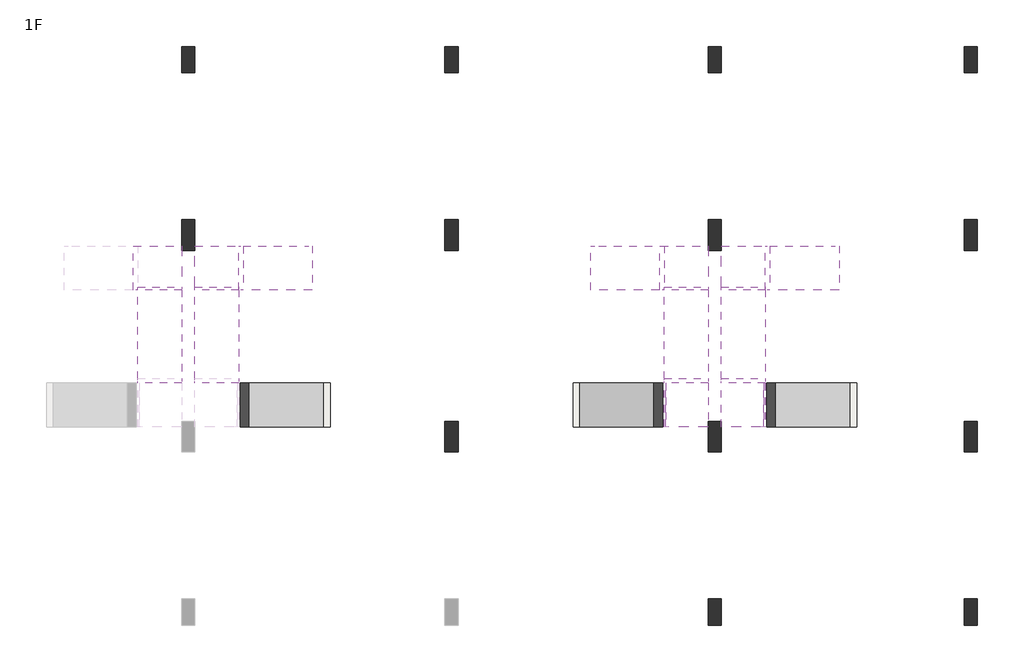
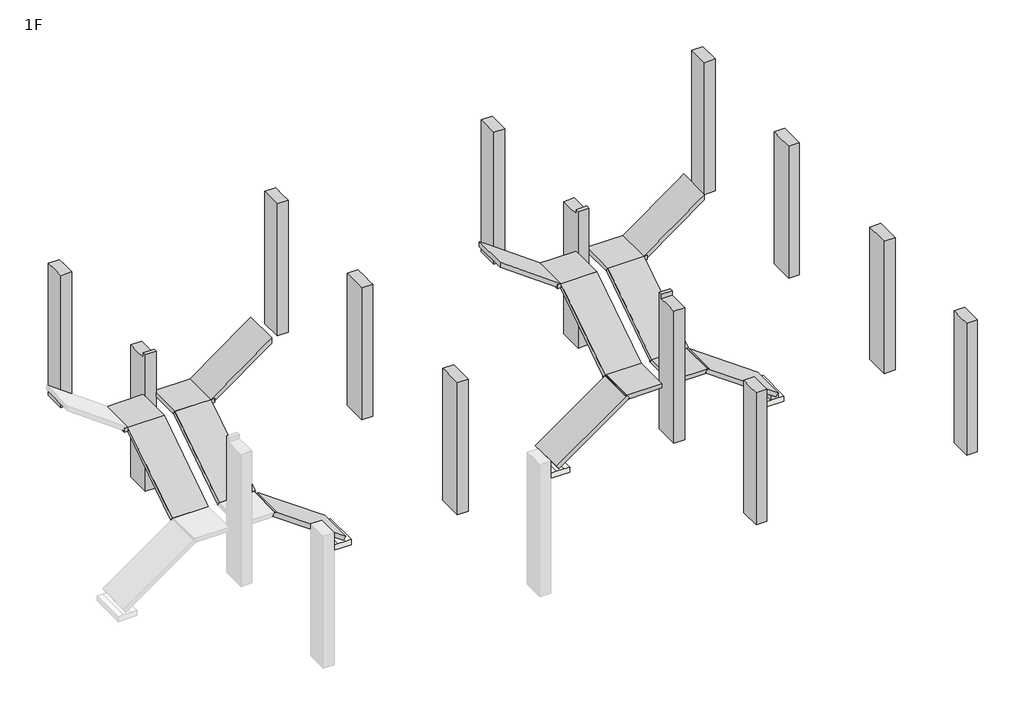
# One storey, part 2 of 2: 17 beams, 13 columns, 3 slabs.
"""IFC4 building model written with IfcOpenShell, lengths in millimetres."""

from ifc_helpers import new_model, si_unit, frame, origin, place, context, project, spatial, polyline, outline, extrude, faceted_brep, element, save

model = new_model("IFC4")

# Units and contexts
model_context = context("Model", 3, world=origin())
ifc_project = project(units=[si_unit("LENGTHUNIT", "METRE", prefix="MILLI")], contexts=[model_context])

# Site, building, storey
site = spatial("IfcSite", under=ifc_project)
building = spatial("IfcBuilding", under=site)
storey = spatial("IfcBuildingStorey", under=building, Name="1F", Elevation=30.0)

# Beams
placement = place(None, origin())
element("IfcBeam", 1, ObjectType="M_Concrete-Rectangular Beam : 1000x120", at=placement, inside=storey, context=model_context, shape_type="Brep", body=[
    faceted_brep([(16700.0000058, 7550.0000002, 2813.0), (17700.0000058, 7550.0000002, 2813.0), (17700.0000058, 7615.755173, 2712.6194379), (16700.0000058, 7615.755173, 2712.6194379), (16700.0000058, 5424.9999998, 1421.0), (16700.0000058, 5490.7551727, 1320.6194379), (17700.0000058, 5490.7551727, 1320.6194379), (17700.0000058, 5424.9999998, 1421.0), (17700.0000058, 5524.9999998, 1343.0518141), (17700.0000058, 7585.8045224, 2693.0), (16700.0000058, 5524.9999998, 1343.0518141), (16700.0000058, 7585.8045224, 2693.0)], [[[0, 1, 2, 3]], [[4, 5, 6, 7]], [[1, 0, 4, 7]], [[2, 1, 7, 6, 8, 9]], [[3, 2, 9, 8, 6, 5, 10, 11]], [[0, 3, 11, 10, 5, 4]]]),
])
element("IfcBeam", 2, ObjectType="M_Concrete-Rectangular Beam : 1000x120", at=placement, inside=storey, context=model_context, shape_type="Brep", body=[
    faceted_brep([(16600.0000058, 7550.0000002, 2813.0), (16600.0000058, 8550.0000002, 2813.0), (16600.0000058, 8550.0000002, 2693.0), (16600.0000058, 7550.0000002, 2693.0), (17700.0000058, 8550.0000002, 2693.0), (17700.0000058, 8550.0000002, 2813.0), (17700.0000058, 7550.0000002, 2813.0), (17700.0000058, 7615.755173, 2712.6194379), (17700.0000058, 7585.8045224, 2693.0), (16700.0000058, 7550.0000002, 2813.0), (16700.0000058, 7585.8045224, 2693.0), (16700.0000058, 7550.0000002, 2693.0), (16700.0000058, 7615.755173, 2712.6194379)], [[[0, 1, 2, 3]], [[4, 5, 6, 7, 8]], [[1, 0, 9, 6, 5]], [[2, 1, 5, 4]], [[3, 2, 4, 8, 10, 11]], [[0, 3, 11, 9]], [[12, 7, 6, 9]], [[7, 12, 10, 8]], [[12, 9, 11, 10]]]),
])
element("IfcBeam", 3, ObjectType="M_Concrete-Rectangular Beam : 1000x120", at=placement, inside=storey, context=model_context, shape_type="Brep", body=[
    faceted_brep([(18969.5227998, 5424.9999998, 1421.3386706), (18969.2824473, 5424.9999998, 1421.0), (18900.072088, 5424.9999998, 1323.4785734), (18900.072088, 4424.9999998, 1323.4785734), (18969.2824473, 4424.9999998, 1421.0), (18969.5227998, 4424.9999998, 1421.3386706), (20930.0000065, 5424.9999998, 30.0), (20930.0000065, 4424.9999998, 30.0), (20860.5492946, 4424.9999998, -67.8600972), (20860.5492946, 5424.9999998, -67.8600972), (18970.0000065, 4424.9999998, 1421.0), (19000.0000058, 4424.9999998, 1399.7091842), (19000.0000058, 5424.9999998, 1399.7091842), (18970.0000065, 5424.9999998, 1421.0), (18931.7457069, 4424.9999998, 1301.0), (18931.7457069, 5424.9999998, 1301.0)], [[[0, 1, 2, 3, 4, 5]], [[6, 7, 8, 9]], [[5, 10, 11, 7, 6, 12, 13, 0]], [[3, 14, 8, 7, 11, 10, 5, 4]], [[2, 15, 9, 8, 14, 3]], [[0, 13, 12, 6, 9, 15, 2, 1]]]),
])
element("IfcBeam", 4, ObjectType="M_Concrete-Rectangular Beam : 1000x120", at=placement, inside=storey, context=model_context, shape_type="Brep", body=[
    faceted_brep([(19000.0000058, 7550.0000002, 2813.0), (19000.0000058, 7615.755173, 2712.6194379), (18000.0000058, 7615.755173, 2712.6194379), (18000.0000058, 7550.0000002, 2813.0), (19000.0000058, 5424.9999998, 1421.0), (18000.0000058, 5424.9999998, 1421.0), (18000.0000058, 5490.7551727, 1320.6194379), (19000.0000058, 5490.7551727, 1320.6194379), (18000.0000058, 7585.8045224, 2693.0), (18000.0000058, 5524.9999998, 1343.0518141), (19000.0000058, 7585.8045224, 2693.0), (19000.0000058, 5524.9999998, 1343.0518141)], [[[0, 1, 2, 3]], [[4, 5, 6, 7]], [[3, 5, 4, 0]], [[2, 8, 9, 6, 5, 3]], [[1, 10, 11, 7, 6, 9, 8, 2]], [[0, 4, 7, 11, 10, 1]]]),
])
element("IfcBeam", 5, ObjectType="M_Concrete-Rectangular Beam : 1000x120", at=placement, inside=storey, context=model_context, shape_type="Brep", body=[
    faceted_brep([(19100.0000058, 8550.0000002, 2813.0), (19100.0000058, 7550.0000002, 2813.0), (19100.0000058, 7550.0000002, 2693.0), (19100.0000058, 8550.0000002, 2693.0), (18000.0000058, 8550.0000002, 2813.0), (18000.0000058, 8550.0000002, 2693.0), (18000.0000058, 7585.8045224, 2693.0), (18000.0000058, 7615.755173, 2712.6194379), (18000.0000058, 7550.0000002, 2813.0), (19000.0000058, 7550.0000002, 2813.0), (19000.0000058, 7550.0000002, 2693.0), (19000.0000058, 7585.8045224, 2693.0), (19000.0000058, 7615.755173, 2712.6194379)], [[[0, 1, 2, 3]], [[4, 5, 6, 7, 8]], [[1, 0, 4, 8, 9]], [[0, 3, 5, 4]], [[3, 2, 10, 11, 6, 5]], [[2, 1, 9, 10]], [[12, 9, 8, 7]], [[12, 7, 6, 11]], [[9, 12, 11, 10]]]),
])
element("IfcBeam", 6, ObjectType="M_Concrete-Rectangular Beam : 1000x120", at=placement, inside=storey, context=model_context, shape_type="Brep", body=[
    faceted_brep([(19000.0000531, 8549.9999993, 2813.0), (19000.0000531, 7549.9999993, 2813.0), (20680.0000464, 7549.9999993, 4030.0), (20680.0000058, 8549.9999993, 4029.9999706), (20500.5423643, 8549.9999993, 3900.0), (19100.0000058, 8549.9999993, 2737.262925), (19100.0000058, 8549.9999993, 2813.0), (20680.0000058, 8549.9999993, 3900.0), (20680.0000058, 8549.9999993, 3881.8224534), (19100.0000058, 7549.9999993, 2737.262925), (20680.0000058, 7549.9999993, 3881.8224534), (19100.0000058, 7549.9999993, 2813.0), (20680.0000058, 7549.9999993, 3900.0)], [[[0, 1, 2, 3, 4]], [[5, 6, 0, 4, 3, 7, 8]], [[9, 5, 8, 10]], [[11, 9, 10, 12, 2, 1]], [[11, 6, 5, 9]], [[6, 11, 1, 0]], [[3, 2, 12, 10, 8, 7]]]),
])
element("IfcBeam", 7, ObjectType="M_Concrete-Rectangular Beam : 1000x120", at=placement, inside=storey, context=model_context, shape_type="Brep", body=[
    faceted_brep([(28730.4772098, 5424.9999998, 1421.3386706), (28730.4772098, 4424.9999998, 1421.3386706), (28730.7175623, 4424.9999998, 1421.0), (28799.9279216, 4424.9999998, 1323.4785734), (28799.9279216, 5424.9999998, 1323.4785734), (28730.7175623, 5424.9999998, 1421.0), (26770.0000031, 5424.9999998, 30.0), (26839.450715, 5424.9999998, -67.8600972), (26839.450715, 4424.9999998, -67.8600972), (26770.0000031, 4424.9999998, 30.0), (28730.0000031, 5424.9999998, 1421.0), (28700.0000039, 5424.9999998, 1399.7091842), (28700.0000039, 4424.9999998, 1399.7091842), (28730.0000031, 4424.9999998, 1421.0), (28768.2543027, 4424.9999998, 1301.0), (28768.2543027, 5424.9999998, 1301.0)], [[[0, 1, 2, 3, 4, 5]], [[6, 7, 8, 9]], [[1, 0, 10, 11, 6, 9, 12, 13]], [[3, 2, 1, 13, 12, 9, 8, 14]], [[4, 3, 14, 8, 7, 15]], [[0, 5, 4, 15, 7, 6, 11, 10]]]),
])
element("IfcBeam", 8, ObjectType="M_Concrete-Rectangular Beam : 1000x120", at=placement, inside=storey, context=model_context, shape_type="Brep", body=[
    faceted_brep([(28700.0000039, 7550.0000002, 2813.0), (29700.0000039, 7550.0000002, 2813.0), (29700.0000039, 7615.755173, 2712.6194379), (28700.0000039, 7615.755173, 2712.6194379), (28700.0000039, 5424.9999998, 1421.0), (28700.0000039, 5490.7551727, 1320.6194379), (29700.0000039, 5490.7551727, 1320.6194379), (29700.0000039, 5424.9999998, 1421.0), (29700.0000039, 5524.9999998, 1343.0518141), (29700.0000039, 7585.8045224, 2693.0), (28700.0000039, 5524.9999998, 1343.0518141), (28700.0000039, 7585.8045224, 2693.0)], [[[0, 1, 2, 3]], [[4, 5, 6, 7]], [[1, 0, 4, 7]], [[2, 1, 7, 6, 8, 9]], [[3, 2, 9, 8, 6, 5, 10, 11]], [[0, 3, 11, 10, 5, 4]]]),
])
element("IfcBeam", 9, ObjectType="M_Concrete-Rectangular Beam : 1000x120", at=placement, inside=storey, context=model_context, shape_type="Brep", body=[
    faceted_brep([(28600.0000039, 7550.0000002, 2813.0), (28600.0000039, 8550.0000002, 2813.0), (28600.0000039, 8550.0000002, 2693.0), (28600.0000039, 7550.0000002, 2693.0), (29700.0000039, 8550.0000002, 2693.0), (29700.0000039, 8550.0000002, 2813.0), (29700.0000039, 7550.0000002, 2813.0), (29700.0000039, 7615.755173, 2712.6194379), (29700.0000039, 7585.8045224, 2693.0), (28700.0000039, 7550.0000002, 2813.0), (28700.0000039, 7585.8045224, 2693.0), (28700.0000039, 7550.0000002, 2693.0), (28700.0000039, 7615.755173, 2712.6194379)], [[[0, 1, 2, 3]], [[4, 5, 6, 7, 8]], [[1, 0, 9, 6, 5]], [[2, 1, 5, 4]], [[3, 2, 4, 8, 10, 11]], [[0, 3, 11, 9]], [[12, 7, 6, 9]], [[7, 12, 10, 8]], [[12, 9, 11, 10]]]),
])
element("IfcBeam", 10, ObjectType="M_Concrete-Rectangular Beam : 1000x120", at=placement, inside=storey, context=model_context, shape_type="Brep", body=[
    faceted_brep([(28699.9999565, 7549.9999993, 2813.0), (28699.9999565, 8549.9999993, 2813.0), (27199.4576453, 8549.9999993, 3900.0), (27019.9999632, 8549.9999993, 4030.0), (27020.000004, 7549.9999993, 4029.9999704), (28600.0000039, 8549.9999993, 2813.0), (28600.0000039, 8549.9999993, 2737.262925), (27020.000004, 8549.9999993, 3881.8224532), (27020.000004, 8549.9999993, 3900.0), (28600.0000039, 7549.9999993, 2737.262925), (27020.000004, 7549.9999993, 3881.8224532), (28600.0000039, 7549.9999993, 2813.0), (27020.000004, 7549.9999993, 3900.0)], [[[0, 1, 2, 3, 4]], [[5, 6, 7, 8, 3, 2, 1]], [[6, 9, 10, 7]], [[9, 11, 0, 4, 12, 10]], [[5, 11, 9, 6]], [[11, 5, 1, 0]], [[4, 3, 8, 7, 10, 12]]]),
])
element("IfcBeam", 11, ObjectType="M_Concrete-Rectangular Beam : 1000x120", at=placement, inside=storey, context=model_context, shape_type="Brep", body=[
    faceted_brep([(29700.0000039, 5524.9999998, 1301.0), (28700.0000039, 5524.9999998, 1301.0), (28700.0000039, 5524.9999998, 1343.0518141), (29700.0000039, 5524.9999998, 1343.0518141), (29700.0000039, 4424.9999998, 1301.0), (29700.0000039, 4424.9999998, 1421.0), (28730.7175623, 4424.9999998, 1421.0), (28799.9279216, 4424.9999998, 1323.4785734), (28768.2543027, 4424.9999998, 1301.0), (28730.0000031, 4424.9999998, 1421.0), (28730.0000031, 5424.9999998, 1421.0), (28700.0000039, 5424.9999998, 1421.0), (28700.0000039, 4424.9999998, 1421.0), (29700.0000039, 5490.7551727, 1320.6194379), (29700.0000039, 5424.9999998, 1421.0), (28768.2543027, 5424.9999998, 1301.0), (28700.0000039, 5424.9999998, 1301.0), (28700.0000039, 5424.9999998, 1399.7091842), (28700.0000039, 4424.9999998, 1399.7091842), (28700.0000039, 5490.7551727, 1320.6194379), (28799.9279216, 5424.9999998, 1323.4785734), (28730.7175623, 5424.9999998, 1421.0)], [[[0, 1, 2, 3]], [[4, 5, 6, 7, 8]], [[9, 10, 11, 12]], [[5, 4, 0, 3, 13, 14]], [[1, 0, 4, 8, 15, 16]], [[17, 18, 12, 11, 19, 2, 1, 16]], [[20, 7, 6, 21]], [[17, 10, 9, 18]], [[7, 20, 15, 8]], [[20, 21, 10, 17, 16, 15]], [[12, 18, 9]], [[13, 19, 11, 10, 21, 14]], [[19, 13, 3, 2]], [[21, 6, 5, 14]]]),
])
element("IfcBeam", 12, ObjectType="M_Concrete-Rectangular Beam : 1000x120", at=placement, inside=storey, context=model_context, shape_type="Brep", body=[
    faceted_brep([(30969.5227979, 5424.9999998, 1421.3386706), (30969.2824454, 5424.9999998, 1421.0), (30900.0720861, 5424.9999998, 1323.4785734), (30900.0720861, 4424.9999998, 1323.4785734), (30969.2824454, 4424.9999998, 1421.0), (30969.5227979, 4424.9999998, 1421.3386706), (32930.0000046, 5424.9999998, 30.0), (32930.0000046, 4424.9999998, 30.0), (32860.5492927, 4424.9999998, -67.8600972), (32860.5492927, 5424.9999998, -67.8600972), (30970.0000046, 4424.9999998, 1421.0), (31000.0000039, 4424.9999998, 1399.7091842), (31000.0000039, 5424.9999998, 1399.7091842), (30970.0000046, 5424.9999998, 1421.0), (30931.745705, 4424.9999998, 1301.0), (32722.6587172, 4424.9999998, 30.0), (30931.745705, 5424.9999998, 1301.0), (32722.6587172, 5424.9999998, 30.0)], [[[0, 1, 2, 3, 4, 5]], [[6, 7, 8, 9]], [[5, 10, 11, 7, 6, 12, 13, 0]], [[3, 14, 15, 8, 7, 11, 10, 5, 4]], [[2, 16, 17, 9, 8, 15, 14, 3]], [[0, 13, 12, 6, 9, 17, 16, 2, 1]]]),
])
element("IfcBeam", 13, ObjectType="M_Concrete-Rectangular Beam : 1000x120", at=placement, inside=storey, context=model_context, shape_type="Brep", body=[
    faceted_brep([(31000.0000039, 7550.0000002, 2813.0), (31000.0000039, 7615.755173, 2712.6194379), (30000.0000039, 7615.755173, 2712.6194379), (30000.0000039, 7550.0000002, 2813.0), (31000.0000039, 5424.9999998, 1421.0), (30000.0000039, 5424.9999998, 1421.0), (30000.0000039, 5490.7551727, 1320.6194379), (31000.0000039, 5490.7551727, 1320.6194379), (30000.0000039, 7585.8045224, 2693.0), (30000.0000039, 5524.9999998, 1343.0518141), (31000.0000039, 7585.8045224, 2693.0), (31000.0000039, 5524.9999998, 1343.0518141)], [[[0, 1, 2, 3]], [[4, 5, 6, 7]], [[3, 5, 4, 0]], [[2, 8, 9, 6, 5, 3]], [[1, 10, 11, 7, 6, 9, 8, 2]], [[0, 4, 7, 11, 10, 1]]]),
])
element("IfcBeam", 14, ObjectType="M_Concrete-Rectangular Beam : 1000x120", at=placement, inside=storey, context=model_context, shape_type="Brep", body=[
    faceted_brep([(31100.0000039, 8550.0000002, 2813.0), (31100.0000039, 7550.0000002, 2813.0), (31100.0000039, 7550.0000002, 2693.0), (31100.0000039, 8550.0000002, 2693.0), (30000.0000039, 8550.0000002, 2813.0), (30000.0000039, 8550.0000002, 2693.0), (30000.0000039, 7585.8045224, 2693.0), (30000.0000039, 7615.755173, 2712.6194379), (30000.0000039, 7550.0000002, 2813.0), (31000.0000039, 7550.0000002, 2813.0), (31000.0000039, 7550.0000002, 2693.0), (31000.0000039, 7585.8045224, 2693.0), (31000.0000039, 7615.755173, 2712.6194379)], [[[0, 1, 2, 3]], [[4, 5, 6, 7, 8]], [[1, 0, 4, 8, 9]], [[0, 3, 5, 4]], [[3, 2, 10, 11, 6, 5]], [[2, 1, 9, 10]], [[12, 9, 8, 7]], [[12, 7, 6, 11]], [[9, 12, 11, 10]]]),
])
element("IfcBeam", 15, ObjectType="M_Concrete-Rectangular Beam : 1000x120", at=placement, inside=storey, context=model_context, shape_type="Brep", body=[
    faceted_brep([(31000.0000512, 8549.9999993, 2813.0), (31000.0000512, 7549.9999993, 2813.0), (32680.0000445, 7549.9999993, 4030.0), (32680.0000108, 8549.9999993, 4029.9999756), (32500.5423624, 8549.9999993, 3900.0), (31100.0000039, 8549.9999993, 2737.262925), (31100.0000039, 8549.9999993, 2813.0), (32680.0000108, 8549.9999993, 3900.0), (32680.0000108, 8549.9999993, 3881.8224584), (31100.0000039, 7549.9999993, 2737.262925), (32680.0000108, 7549.9999993, 3881.8224584), (31100.0000039, 7549.9999993, 2813.0), (32680.0000108, 7549.9999993, 3900.0)], [[[0, 1, 2, 3, 4]], [[5, 6, 0, 4, 3, 7, 8]], [[9, 5, 8, 10]], [[11, 9, 10, 12, 2, 1]], [[11, 6, 5, 9]], [[6, 11, 1, 0]], [[3, 2, 12, 10, 8, 7]]]),
])
element("IfcBeam", 16, ObjectType="M_Concrete-Rectangular Beam : 1000x120", at=placement, inside=storey, context=model_context, shape_type="Brep", body=[
    faceted_brep([(31000.0000039, 5524.9999998, 1301.0), (30000.0000039, 5524.9999998, 1301.0), (30000.0000039, 5524.9999998, 1343.0518141), (31000.0000039, 5524.9999998, 1343.0518141), (30000.0000039, 4424.9999998, 1421.0), (30000.0000039, 4424.9999998, 1301.0), (30931.745705, 4424.9999998, 1301.0), (30900.0720861, 4424.9999998, 1323.4785734), (30969.2824454, 4424.9999998, 1421.0), (30970.0000046, 5424.9999998, 1421.0), (30970.0000046, 4424.9999998, 1421.0), (31000.0000039, 4424.9999998, 1421.0), (31000.0000039, 5424.9999998, 1421.0), (30000.0000039, 5424.9999998, 1421.0), (30000.0000039, 5490.7551727, 1320.6194379), (31000.0000039, 5424.9999998, 1301.0), (30931.745705, 5424.9999998, 1301.0), (31000.0000039, 4424.9999998, 1399.7091842), (31000.0000039, 5424.9999998, 1399.7091842), (31000.0000039, 5490.7551727, 1320.6194379), (30900.0720861, 5424.9999998, 1323.4785734), (30969.2824454, 5424.9999998, 1421.0)], [[[0, 1, 2, 3]], [[4, 5, 6, 7, 8]], [[9, 10, 11, 12]], [[5, 4, 13, 14, 2, 1]], [[1, 0, 15, 16, 6, 5]], [[17, 18, 15, 0, 3, 19, 12, 11]], [[7, 20, 21, 8]], [[10, 9, 18, 17]], [[20, 7, 6, 16]], [[21, 20, 16, 15, 18, 9]], [[17, 11, 10]], [[19, 14, 13, 21, 9, 12]], [[14, 19, 3, 2]], [[8, 21, 13, 4]]]),
])
element("IfcBeam", 17, ObjectType="M_Concrete-Rectangular Beam : 220x300", at=placement, inside=storey, context=model_context, shape_type="SweptSolid", body=[
    extrude(outline(polyline([(30.0, 32710.0000046), (-120.0, 32710.0000046), (-120.0, 32930.0000046), (30.0, 32930.0000046), (-67.8600972, 32860.5492927), (30.0, 32722.6587172), (30.0, 32710.0000046)])), frame((0.0, 4424.9999998, 0.0), z_axis=(0.0, 1.0, 0.0), x_axis=(0.0, 0.0, 1.0)), (0.0, 0.0, 1.0), 1000.0),
])

# Columns
element("IfcColumn", 18, ObjectType="M_Concrete-Rectangular-Column : 300x600", at=placement, inside=storey, context=model_context, shape_type="Brep", body=[
    faceted_brep([(18000.0000058, 13100.0000003, 30.0), (18000.0000058, 12500.0000003, 30.0), (17700.0000058, 12500.0000003, 30.0), (17700.0000058, 13100.0000003, 30.0), (18000.0000058, 13100.0000003, 3900.0), (18000.0000058, 12799.9999993, 3900.0), (18000.0000058, 12500.0000003, 3900.0), (17700.0000058, 12500.0000003, 3900.0), (17700.0000058, 12799.9999993, 3900.0), (17700.0000058, 13100.0000003, 3900.0), (17700.0000058, 13100.0000003, 3330.0)], [[[0, 1, 2, 3]], [[1, 0, 4, 5, 6]], [[2, 1, 6, 7]], [[3, 2, 7, 8, 9, 10]], [[0, 3, 10, 9, 4]], [[6, 5, 4, 9, 8, 7]]]),
])
element("IfcColumn", 19, ObjectType="M_Concrete-Rectangular-Column : 300x600", at=placement, inside=storey, context=model_context, shape_type="Brep", body=[
    faceted_brep([(24000.0000047, 13100.0000003, 30.0), (24000.0000047, 12500.0000003, 30.0), (23700.0000047, 12500.0000003, 30.0), (23700.0000047, 13100.0000003, 30.0), (24000.0000047, 13100.0000003, 3900.0), (24000.0000047, 12799.9999993, 3900.0), (24000.0000047, 12500.0000003, 3900.0), (23700.0000047, 12500.0000003, 3900.0), (23700.0000047, 12799.9999993, 3900.0), (23700.0000047, 13100.0000003, 3900.0), (23700.0000047, 13100.0000003, 3330.0)], [[[0, 1, 2, 3]], [[1, 0, 4, 5, 6]], [[2, 1, 6, 7]], [[3, 2, 7, 8, 9, 10]], [[0, 3, 10, 9, 4]], [[6, 5, 4, 9, 8, 7]]]),
])
element("IfcColumn", 20, ObjectType="M_Concrete-Rectangular-Column : 300x600", at=placement, inside=storey, context=model_context, shape_type="Brep", body=[
    faceted_brep([(30000.0000039, 499.9999998, 30.0), (30000.0000039, -100.0000002, 30.0), (29700.0000039, -100.0000002, 30.0), (29700.0000039, 499.9999998, 30.0), (30000.0000039, 499.9999998, 3900.0), (30000.0000039, 200.000001, 3900.0), (30000.0000039, -100.0000002, 3900.0), (29700.0000039, -100.0000002, 3900.0), (29700.0000039, -100.0000002, 3330.0), (29700.0000039, 200.000001, 3900.0), (29700.0000039, 499.9999998, 3900.0)], [[[0, 1, 2, 3]], [[1, 0, 4, 5, 6]], [[2, 1, 6, 7, 8]], [[3, 2, 8, 7, 9, 10]], [[0, 3, 10, 4]], [[6, 5, 4, 10, 9, 7]]]),
])
element("IfcColumn", 21, ObjectType="M_Concrete-Rectangular-Column : 300x600", at=placement, inside=storey, context=model_context, shape_type="Brep", body=[
    faceted_brep([(30000.0000039, 13100.0000003, 30.0), (30000.0000039, 12500.0000003, 30.0), (29700.0000039, 12500.0000003, 30.0), (29700.0000039, 13100.0000003, 30.0), (30000.0000039, 13100.0000003, 3900.0), (30000.0000039, 12799.9999993, 3900.0), (30000.0000039, 12500.0000003, 3900.0), (29700.0000039, 12500.0000003, 3900.0), (29700.0000039, 12799.9999993, 3900.0), (29700.0000039, 13100.0000003, 3900.0), (29700.0000039, 13100.0000003, 3330.0)], [[[0, 1, 2, 3]], [[1, 0, 4, 5, 6]], [[2, 1, 6, 7]], [[3, 2, 7, 8, 9, 10]], [[0, 3, 10, 9, 4]], [[6, 5, 4, 9, 8, 7]]]),
])
element("IfcColumn", 22, ObjectType="M_Concrete-Rectangular-Column : 300x600", at=placement, inside=storey, context=model_context, shape_type="Brep", body=[
    faceted_brep([(35835.035019, 499.9999998, 30.0), (35835.035019, -100.0000002, 30.0), (35535.035019, -100.0000002, 30.0), (35535.035019, 499.9999998, 30.0), (35835.035019, 499.9999998, 3630.0), (35835.035019, 499.9999998, 3900.0), (35835.035019, -100.0000002, 3900.0), (35835.035019, -100.0000002, 3330.0), (35535.035019, -100.0000002, 3900.0), (35535.035019, -100.0000002, 3330.0), (35535.035019, 200.000001, 3900.0), (35535.035019, 499.9999998, 3900.0), (35535.035019, 499.9999998, 3630.0)], [[[0, 1, 2, 3]], [[1, 0, 4, 5, 6, 7]], [[2, 1, 7, 6, 8, 9]], [[3, 2, 9, 8, 10, 11, 12]], [[0, 3, 12, 11, 5, 4]], [[6, 5, 11, 10, 8]]]),
])
element("IfcColumn", 23, ObjectType="M_Concrete-Rectangular-Column : 300x600", at=placement, inside=storey, context=model_context, shape_type="Brep", body=[
    faceted_brep([(35835.035019, 13100.0000003, 30.0), (35835.035019, 12500.0000003, 30.0), (35535.035019, 12500.0000003, 30.0), (35535.035019, 13100.0000003, 30.0), (35835.035019, 13100.0000003, 3330.0), (35835.035019, 13100.0000003, 3900.0), (35835.035019, 12500.0000003, 3900.0), (35835.035019, 12500.0000003, 3630.0), (35535.035019, 12500.0000003, 3900.0), (35535.035019, 12500.0000003, 3630.0), (35535.035019, 12799.9999993, 3900.0), (35535.035019, 13100.0000003, 3900.0), (35535.035019, 13100.0000003, 3330.0)], [[[0, 1, 2, 3]], [[1, 0, 4, 5, 6, 7]], [[2, 1, 7, 6, 8, 9]], [[3, 2, 9, 8, 10, 11, 12]], [[0, 3, 12, 11, 5, 4]], [[6, 5, 11, 10, 8]]]),
])
element("IfcColumn", 24, ObjectType="M_Concrete-Rectangular-Column : 300x700", at=placement, inside=storey, context=model_context, shape_type="Brep", body=[
    faceted_brep([(24000.0000047, 4550.0000002, 30.0), (24000.0000047, 3850.0000002, 30.0), (23700.0000047, 3850.0000002, 30.0), (23700.0000047, 4550.0000002, 30.0), (24000.0000047, 4550.0000002, 3900.0), (24000.0000047, 4449.9999998, 3900.0), (24000.0000047, 4149.9999998, 3900.0), (24000.0000047, 3850.0000002, 3900.0), (23700.0000047, 3850.0000002, 3900.0), (23700.0000047, 4149.9999998, 3900.0), (23700.0000047, 4449.9999998, 3900.0), (23700.0000047, 4550.0000002, 3900.0)], [[[0, 1, 2, 3]], [[1, 0, 4, 5, 6, 7]], [[2, 1, 7, 8]], [[3, 2, 8, 9, 10, 11]], [[0, 3, 11, 4]], [[7, 6, 5, 4, 11, 10, 9, 8]]]),
])
element("IfcColumn", 25, ObjectType="M_Concrete-Rectangular-Column : 300x700", at=placement, inside=storey, context=model_context, shape_type="Brep", body=[
    faceted_brep([(18000.0000058, 9149.9985388, 30.0), (18000.0000058, 8449.9985388, 30.0), (17700.0000058, 8449.9985388, 30.0), (17700.0000058, 9149.9985388, 30.0), (18000.0000058, 9149.9985388, 3900.0), (18000.0000058, 8849.9999993, 3900.0), (18000.0000058, 8549.9999993, 3900.0), (18000.0000058, 8549.9999993, 4030.0), (18000.0000058, 8449.9985388, 4030.0), (17700.0000058, 8449.9985388, 4030.0), (17700.0000058, 8549.9999993, 4030.0), (17700.0000058, 8549.9999993, 3900.0), (17700.0000058, 8849.9999993, 3900.0), (17700.0000058, 9149.9985388, 3900.0)], [[[0, 1, 2, 3]], [[1, 0, 4, 5, 6, 7, 8]], [[2, 1, 8, 9]], [[3, 2, 9, 10, 11, 12, 13]], [[0, 3, 13, 4]], [[9, 8, 7, 10]], [[11, 6, 5, 4, 13, 12]], [[6, 11, 10, 7]]]),
])
element("IfcColumn", 26, ObjectType="M_Concrete-Rectangular-Column : 300x700", at=placement, inside=storey, context=model_context, shape_type="Brep", body=[
    faceted_brep([(24000.0000047, 9149.9985388, 30.0), (24000.0000047, 8449.9985388, 30.0), (23700.0000047, 8449.9985388, 30.0), (23700.0000047, 9149.9985388, 30.0), (24000.0000047, 9149.9985388, 3900.0), (24000.0000047, 8849.9999993, 3900.0), (24000.0000047, 8549.9999993, 3900.0), (24000.0000047, 8449.9985388, 3900.0), (23700.0000047, 8449.9985388, 3900.0), (23700.0000047, 8549.9999993, 3900.0), (23700.0000047, 8849.9999993, 3900.0), (23700.0000047, 9149.9985388, 3900.0)], [[[0, 1, 2, 3]], [[1, 0, 4, 5, 6, 7]], [[2, 1, 7, 8]], [[3, 2, 8, 9, 10, 11]], [[0, 3, 11, 4]], [[7, 6, 5, 4, 11, 10, 9, 8]]]),
])
element("IfcColumn", 27, ObjectType="M_Concrete-Rectangular-Column : 300x700", at=placement, inside=storey, context=model_context, shape_type="Brep", body=[
    faceted_brep([(30000.0000039, 4550.0000002, 30.0), (30000.0000039, 3850.0000002, 30.0), (29700.0000039, 3850.0000002, 30.0), (29700.0000039, 4550.0000002, 30.0), (30000.0000039, 4550.0000002, 4030.0), (30000.0000039, 4450.0000002, 4030.0), (30000.0000039, 4450.0000002, 3900.0), (30000.0000039, 4149.9999998, 3900.0), (30000.0000039, 3850.0000002, 3900.0), (29700.0000039, 3850.0000002, 3900.0), (29700.0000039, 4149.9999998, 3900.0), (29700.0000039, 4450.0000002, 3900.0), (29700.0000039, 4450.0000002, 4030.0), (29700.0000039, 4550.0000002, 4030.0)], [[[0, 1, 2, 3]], [[1, 0, 4, 5, 6, 7, 8]], [[2, 1, 8, 9]], [[3, 2, 9, 10, 11, 12, 13]], [[0, 3, 13, 4]], [[4, 13, 12, 5]], [[6, 11, 10, 9, 8, 7]], [[11, 6, 5, 12]]]),
])
element("IfcColumn", 28, ObjectType="M_Concrete-Rectangular-Column : 300x700", at=placement, inside=storey, context=model_context, shape_type="Brep", body=[
    faceted_brep([(30000.0000039, 9149.9985388, 30.0), (30000.0000039, 8449.9985388, 30.0), (29700.0000039, 8449.9985388, 30.0), (29700.0000039, 9149.9985388, 30.0), (30000.0000039, 9149.9985388, 3900.0), (30000.0000039, 8849.9999993, 3900.0), (30000.0000039, 8549.9999993, 3900.0), (30000.0000039, 8549.9999993, 4030.0), (30000.0000039, 8449.9985388, 4030.0), (29700.0000039, 8449.9985388, 4030.0), (29700.0000039, 8549.9999993, 4030.0), (29700.0000039, 8549.9999993, 3900.0), (29700.0000039, 8849.9999993, 3900.0), (29700.0000039, 9149.9985388, 3900.0)], [[[0, 1, 2, 3]], [[1, 0, 4, 5, 6, 7, 8]], [[2, 1, 8, 9]], [[3, 2, 9, 10, 11, 12, 13]], [[0, 3, 13, 4]], [[9, 8, 7, 10]], [[11, 6, 5, 4, 13, 12]], [[6, 11, 10, 7]]]),
])
element("IfcColumn", 29, ObjectType="M_Concrete-Rectangular-Column : 300x700", at=placement, inside=storey, context=model_context, shape_type="Brep", body=[
    faceted_brep([(35835.035019, 4550.0000002, 30.0), (35835.035019, 3850.0000002, 30.0), (35535.035019, 3850.0000002, 30.0), (35535.035019, 4550.0000002, 30.0), (35835.035019, 4550.0000002, 3630.0), (35835.035019, 4550.0000002, 3900.0), (35835.035019, 3850.0000002, 3900.0), (35835.035019, 3850.0000002, 3630.0), (35535.035019, 3850.0000002, 3900.0), (35535.035019, 3850.0000002, 3630.0), (35535.035019, 4149.9999998, 3900.0), (35535.035019, 4449.9999998, 3900.0), (35535.035019, 4550.0000002, 3900.0), (35535.035019, 4550.0000002, 3630.0)], [[[0, 1, 2, 3]], [[1, 0, 4, 5, 6, 7]], [[2, 1, 7, 6, 8, 9]], [[3, 2, 9, 8, 10, 11, 12, 13]], [[0, 3, 13, 12, 5, 4]], [[6, 5, 12, 11, 10, 8]]]),
])
element("IfcColumn", 30, ObjectType="M_Concrete-Rectangular-Column : 300x700", at=placement, inside=storey, context=model_context, shape_type="Brep", body=[
    faceted_brep([(35835.035019, 9149.9985388, 30.0), (35835.035019, 8449.9985388, 30.0), (35535.035019, 8449.9985388, 30.0), (35535.035019, 9149.9985388, 30.0), (35835.035019, 9149.9985388, 3630.0), (35835.035019, 9149.9985388, 3900.0), (35835.035019, 8449.9985388, 3900.0), (35835.035019, 8449.9985388, 3630.0), (35535.035019, 8449.9985388, 3900.0), (35535.035019, 8449.9985388, 3630.0), (35535.035019, 8549.9999993, 3900.0), (35535.035019, 8849.9999993, 3900.0), (35535.035019, 9149.9985388, 3900.0), (35535.035019, 9149.9985388, 3630.0)], [[[0, 1, 2, 3]], [[1, 0, 4, 5, 6, 7]], [[2, 1, 7, 6, 8, 9]], [[3, 2, 9, 8, 10, 11, 12, 13]], [[0, 3, 13, 12, 5, 4]], [[6, 5, 12, 11, 10, 8]]]),
])

# Slabs
element("IfcSlab", 31, ObjectType="Mong bang-lech tam : 520x300", at=placement, inside=storey, context=model_context, shape_type="SweptSolid", body=[
    extrude(outline(polyline([(-120.0, 20930.0000065), (-120.0, 20710.0000065), (-120.0, 20560.0000065), (-270.0, 20560.0000065), (-270.0, 21080.0000065), (-120.0, 21080.0000065), (-120.0, 20930.0000065)])), frame((0.0, 4424.9999998, 0.0), z_axis=(0.0, 1.0, 0.0), x_axis=(0.0, 0.0, 1.0)), (0.0, 0.0, 1.0), 1000.0),
])
element("IfcSlab", 32, ObjectType="Mong bang-lech tam : 520x300", at=placement, inside=storey, context=model_context, shape_type="SweptSolid", body=[
    extrude(outline(polyline([(-120.0, 26770.0000031), (-120.0, 26620.0000031), (-270.0, 26620.0000031), (-270.0, 27140.0000031), (-120.0, 27140.0000031), (-120.0, 26990.0000031), (-120.0, 26770.0000031)])), frame((0.0, 4424.9999998, 0.0), z_axis=(0.0, 1.0, 0.0), x_axis=(0.0, 0.0, 1.0)), (0.0, 0.0, 1.0), 1000.0),
])
element("IfcSlab", 33, ObjectType="Mong bang-lech tam : 520x300", at=placement, inside=storey, context=model_context, shape_type="SweptSolid", body=[
    extrude(outline(polyline([(-120.0, 32930.0000046), (-120.0, 32710.0000046), (-120.0, 32560.0000046), (-270.0, 32560.0000046), (-270.0, 33080.0000046), (-120.0, 33080.0000046), (-120.0, 32930.0000046)])), frame((0.0, 4424.9999998, 0.0), z_axis=(0.0, 1.0, 0.0), x_axis=(0.0, 0.0, 1.0)), (0.0, 0.0, 1.0), 1000.0),
])

save(model, "model.ifc")

# Revit data of these elements
# Type "M_Concrete-Rectangular Beam : 1000x120"
#   Length [instance default] = 1524 mm
#   b = 1000 mm
#   h = 120 mm
#   Structural Material [instance default] = Concrete, Cast-in-Place gray
#   Assembly Code = ""
# Type "M_Concrete-Rectangular Beam : 220x300"
#   Length [instance default] = 1524 mm
#   b = 220 mm
#   h = 300 mm
#   Structural Material [instance default] = Concrete, Cast-in-Place gray
#   Assembly Code = ""
# Type "M_Concrete-Rectangular-Column : 300x600"
#   b = 300 mm
#   h = 600 mm
#   Structural Material [instance default] = Concrete, Cast-in-Place gray
# Type "M_Concrete-Rectangular-Column : 300x700"
#   b = 300 mm
#   h = 700 mm
#   Structural Material [instance default] = Concrete, Cast-in-Place gray
# Type "Mong bang-lech tam : 520x300"
#   Length = 1000 mm
#   Lech Tam (E) = 0 mm
#   Foundation Thickness = 150 mm
#   Foundation (h2) = 150 mm
#   Foundation (h1) = 0 mm
#   Be Rong Dam (b) = 220 mm
#   Be Rong Dai Mong (B) = 520 mm
#   Structural Material [instance default] = Concrete, Cast-in-Place gray
#   Width = 0
#   Assembly Code = ""
# Elements 1, 2, 4, 5, 6, 8, 9, 10, 11, 13, 14, 15, 16 (IfcBeam, "M_Concrete-Rectangular Beam : 1000x120")
#   COF_GEN__Name = "STAIR"
#   Structural Material = Concrete, Cast-in-Place gray
#   Phase Created = New Construction
#   Materials on its faces: "Concrete, Cast-in-Place gray"
# Elements 3, 7, 12 (IfcBeam, "M_Concrete-Rectangular Beam : 1000x120")
#   Comments = ""
#   COF_GEN__Name = "STAIR"
#   Structural Material = Concrete, Cast-in-Place gray
#   Phase Created = New Construction
#   Materials on its faces: "Concrete, Cast-in-Place gray"
# Element 17 (IfcBeam, "M_Concrete-Rectangular Beam : 220x300")
#   Comments = ""
#   Structural Material = Concrete, Cast-in-Place gray
#   Phase Created = New Construction
#   Materials on its faces: "Concrete, Cast-in-Place gray"
# Element 18 (IfcColumn, "M_Concrete-Rectangular-Column : 300x600")
#   Comments = ""
#   COF_CON__WorkItemNumber = "SH3-A-02F"
#   COF_GEN__Name = "C2"
#   Structural Material = Concrete, Cast-in-Place gray
#   Phase Created = New Construction
#   Materials on its faces: "Concrete, Cast-in-Place gray"
# Elements 19, 20, 21, 22, 23 (IfcColumn, "M_Concrete-Rectangular-Column : 300x600")
#   Comments = ""
#   COF_CON__WorkItemNumber = "SH3-A-02F"
#   COF_GEN__Name = "C1"
#   Structural Material = Concrete, Cast-in-Place gray
#   Phase Created = New Construction
#   Materials on its faces: "Concrete, Cast-in-Place gray"
# Elements 24, 26 (IfcColumn, "M_Concrete-Rectangular-Column : 300x700")
#   Comments = ""
#   COF_CON__WorkItemNumber = "SH3-A-02F"
#   COF_GEN__Name = "C5"
#   Structural Material = Concrete, Cast-in-Place gray
#   Phase Created = New Construction
#   Materials on its faces: "Concrete, Cast-in-Place gray"
# Element 25 (IfcColumn, "M_Concrete-Rectangular-Column : 300x700")
#   Comments = ""
#   COF_CON__WorkItemNumber = "SH3-A-02F"
#   COF_GEN__Name = "C6"
#   Structural Material = Concrete, Cast-in-Place gray
#   Phase Created = New Construction
#   Materials on its faces: "Concrete, Cast-in-Place gray"
# Elements 27, 28 (IfcColumn, "M_Concrete-Rectangular-Column : 300x700")
#   Comments = ""
#   COF_CON__WorkItemNumber = "SH3-A-02F"
#   COF_GEN__Name = "C4"
#   Structural Material = Concrete, Cast-in-Place gray
#   Phase Created = New Construction
#   Materials on its faces: "Concrete, Cast-in-Place gray"
# Elements 29, 30 (IfcColumn, "M_Concrete-Rectangular-Column : 300x700")
#   Comments = ""
#   COF_CON__WorkItemNumber = "SH3-A-02F"
#   COF_GEN__Name = "C3"
#   Structural Material = Concrete, Cast-in-Place gray
#   Phase Created = New Construction
#   Materials on its faces: "Concrete, Cast-in-Place gray"
# Elements 31, 32, 33 (IfcSlab, "Mong bang-lech tam : 520x300")
#   Comments = ""
#   COF_GEN__Name = "DCT"
#   Structural Material = Concrete, Cast-in-Place gray
#   Phase Created = New Construction
#   Materials on its faces: "Concrete, Cast-in-Place gray"
# Materials
#   "Concrete, Cast-in-Place gray": class "Concrete", colour RGB 207 208 204, transparency 0, Description = "Cast-in-place concrete", Cost = 0
